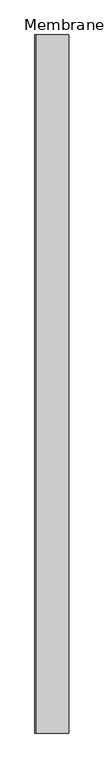
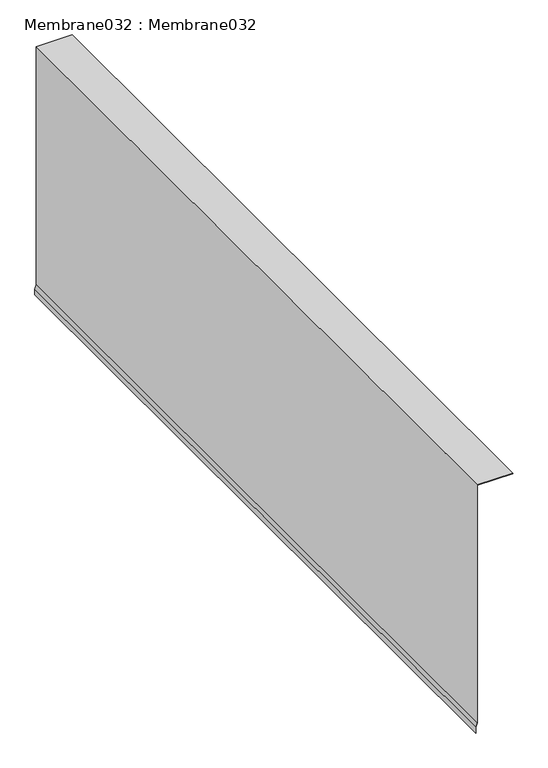
"""IFC4 building model written with IfcOpenShell, lengths in millimetres: proxy geometry, Membrane032 : Membrane032."""

from ifc_helpers import new_model, si_unit, frame, origin, place, context, project, spatial, polyline, outline, extrude, source, transform, mapped, element, save


def membrane032_membrane032_f9e2c576(model_context):
    return source(origin(), model_context, "Body", "SweptSolid", [
        extrude(outline(polyline([(40237.828125, -2674.0896171), (40237.828125, -2767.6617221), (39579.4993977, -2767.6617221), (39568.2741325, -2771.7473845), (39552.6918208, -2771.7473845), (39552.6918208, -2770.7473845), (39568.0978055, -2770.7473845), (39579.3230707, -2766.6617221), (40236.828125, -2766.6617221), (40236.828125, -2674.0896171), (40237.828125, -2674.0896171)])), frame((0.0, -1052.8906574, 0.0), z_axis=(0.0, 1.0, 0.0), x_axis=(0.0, 0.0, 1.0)), (0.0, 0.0, 1.0), 2000.0),
    ])


if __name__ == "__main__":
    model = new_model("IFC4")
    model_context = context("Model", 3, world=origin())
    ifc_project = project(units=[si_unit("LENGTHUNIT", "METRE", prefix="MILLI")], contexts=[model_context])
    site = spatial("IfcSite", under=ifc_project)
    building = spatial("IfcBuilding", under=site)
    placement = place(None, origin())
    membrane032_membrane032_shape = membrane032_membrane032_f9e2c576(model_context)
    element("IfcBuildingElementProxy", 1, Name="Membrane032 : Membrane032", ObjectType="Membrane032 : Membrane032", at=placement, inside=building, context=model_context, shape_type="MappedRepresentation", body=[
        mapped(membrane032_membrane032_shape, transform((0.0, 0.0, 0.0), x_axis=(1.0, 0.0, 0.0), y_axis=(0.0, 1.0, 0.0), z_axis=(0.0, 0.0, 1.0))),
    ])
    save(model, "model.ifc")

# Revit data of these elements
# Type "Membrane032 : Membrane032"
#   NameOverride = "Membrane032"
# Element 1 (IfcBuildingElementProxy, "Membrane032 : Membrane032")
#   Materials on its faces: "2 LAYERS NO. 30 ASTM D226 ASPHALT SATURATED ORGANIC FELT"
# Materials
#   "2 LAYERS NO. 30 ASTM D226 ASPHALT SATURATED ORGANIC FELT": class "Unassigned", colour RGB 46 171 0, transparency 0
